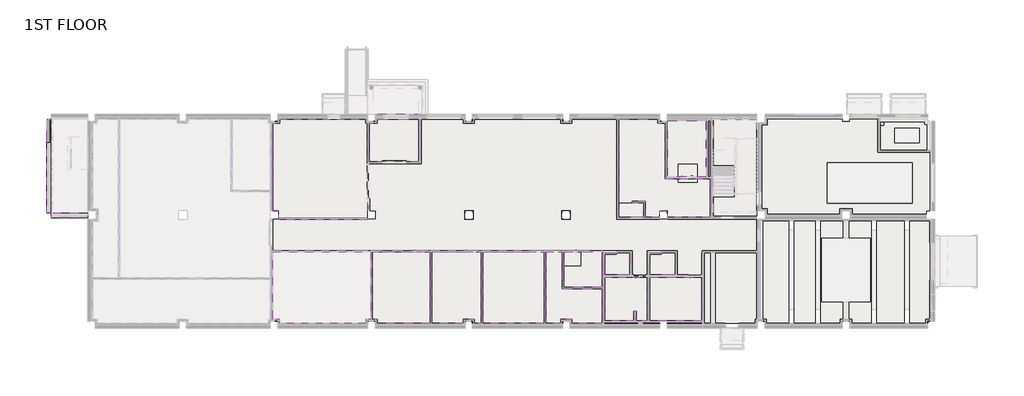
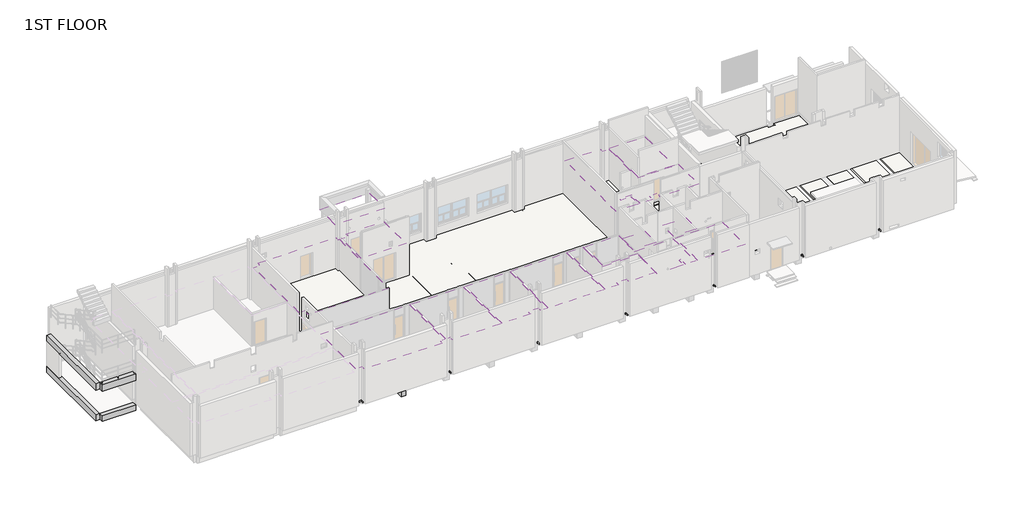
# One storey, part 8 of 15: 26 slabs, 15 coverings, 5 beams.
"""IFC4 building model written with IfcOpenShell, lengths in millimetres."""

from ifc_helpers import new_model, si_unit, frame, origin, place, context, project, spatial, polyline, outline, extrude, faceted_brep, element, save

model = new_model("IFC4")

# Units and contexts
model_context = context("Model", 3, world=origin())
ifc_project = project(units=[si_unit("LENGTHUNIT", "METRE", prefix="MILLI")], contexts=[model_context])

# Site, building, storey
site = spatial("IfcSite", under=ifc_project)
building = spatial("IfcBuilding", under=site)
storey = spatial("IfcBuildingStorey", under=building, Name="1ST FLOOR", Elevation=4800.0)

# Beams
placement = place(None, origin())
element("IfcBeam", 1, ObjectType="RC Beam_Rectangular : H_SB_AR S16_TG-UG_450x800_1B1A", at=placement, inside=storey, context=model_context, shape_type="Brep", body=[
    faceted_brep([(18775.0, -16900.0, 4800.0), (19225.0, -16900.0, 4800.0), (19225.0, -8350.0, 4800.0), (18775.0, -8350.0, 4800.0), (19225.0, -16900.0, 4650.0), (19225.0, -16900.0, 4000.0), (19225.0, -8350.0, 4000.0), (19225.0, -8350.0, 4650.0), (18775.0, -16900.0, 4000.0), (18775.0, -8350.0, 4000.0), (18775.0, -8350.0, 4650.0), (18775.0, -16900.0, 4650.0)], [[[0, 1, 2, 3]], [[2, 1, 4, 5, 6, 7]], [[5, 8, 9, 6]], [[0, 3, 10, 9, 8, 11]], [[1, 0, 11, 8, 5, 4]], [[3, 2, 7, 6, 9, 10]]]),
])
element("IfcBeam", 2, ObjectType="RC Beam_Rectangular : H_SB_AR S16_RC Beam-AG_400x530_SG1A", at=placement, inside=storey, context=model_context, shape_type="Brep", body=[
    faceted_brep([(-300.0, -8200.0, 4630.0), (-300.0, -7800.0, 4630.0), (-3300.0, -7800.0, 4630.0), (-3300.0, -8200.0, 4630.0), (-300.0, -8200.0, 4100.0), (-3300.0, -8200.0, 4100.0), (-300.0, -7800.0, 4100.0), (-3300.0, -7800.0, 4100.0), (-300.0, -7800.0, 4430.0), (-3300.0, -7800.0, 4430.0)], [[[0, 1, 2, 3]], [[4, 0, 3, 5]], [[6, 4, 5, 7]], [[1, 8, 6, 7, 9, 2]], [[1, 0, 4, 6, 8]], [[2, 9, 7, 5, 3]]]),
])
element("IfcBeam", 3, ObjectType="RC Beam_Rectangular : H_SB_AR S16_RC Beam-AG_400x600_SG2", at=placement, inside=storey, context=model_context, shape_type="Brep", body=[
    faceted_brep([(-3700.0, -7800.0, 4630.0), (-3300.0, -7800.0, 4630.0), (-3300.0, -100.0, 4630.0), (-3450.0, -100.0, 4630.0), (-3700.0, -100.0, 4630.0), (-3700.0, -2000.0, 4630.0), (-3700.0, -7800.0, 4030.0), (-3700.0, -100.0, 4030.0), (-3300.0, -7800.0, 4030.0), (-3300.0, -100.0, 4030.0), (-3300.0, -7800.0, 4430.0), (-3300.0, -100.0, 4430.0)], [[[0, 1, 2, 3, 4, 5]], [[6, 0, 5, 4, 7]], [[8, 6, 7, 9]], [[1, 10, 8, 9, 11, 2]], [[1, 0, 6, 8, 10]], [[2, 11, 9, 7, 4, 3]]]),
])
element("IfcBeam", 4, ObjectType="RC Beam_Rectangular : H_SB_AR S16_RC Beam-AG_400x600_SWG2", at=placement, inside=storey, context=model_context, shape_type="Brep", body=[
    faceted_brep([(-3300.0, -100.0, 7590.0), (-3450.0, -100.0, 7590.0), (-3700.0, -100.0, 7590.0), (-3700.0, -2000.0, 7590.0), (-3700.0, -7800.0, 7590.0), (-3300.0, -7800.0, 7590.0), (-3300.0, -100.0, 6990.0), (-3300.0, -7800.0, 6990.0), (-3700.0, -100.0, 6990.0), (-3450.0, -100.0, 6990.0), (-3700.0, -7800.0, 6990.0), (-3700.0, -2000.0, 6990.0)], [[[0, 1, 2, 3, 4, 5]], [[6, 0, 5, 7]], [[8, 9, 6, 7, 10, 11]], [[2, 8, 11, 10, 4, 3]], [[4, 10, 7, 5]], [[2, 1, 0, 6, 9, 8]]]),
])
element("IfcBeam", 5, ObjectType="RC Beam_Rectangular : H_SB_AR S16_RC Beam-AG_400x600_SG1", at=placement, inside=storey, context=model_context, shape_type="SweptSolid", body=[
    extrude(outline(polyline([(-300.0, -7800.0), (-300.0, -8200.0), (-3300.0, -8200.0), (-3300.0, -7800.0), (-300.0, -7800.0)])), frame((0.0, 0.0, 6990.0), z_axis=(0.0, 0.0, 1.0), x_axis=(1.0, 0.0, 0.0)), (0.0, 0.0, 1.0), 600.0),
])

# Coverings
element("IfcCovering", 6, ObjectType="H_CE_AR_B09_2L Gypsum Board_T Bar_9T_C4", at=placement, inside=storey, context=model_context, shape_type="SweptSolid", body=[
    extrude(outline(polyline([(22536.0, -114.0), (22536.0, -464.0), (22649.9999955, -464.0), (22649.9999955, -8250.0), (15400.0000001, -8250.0), (15400.0000001, -7650.0), (14886.0, -7650.0), (14886.0, -464.0), (15464.0, -464.0), (15464.0, -114.0), (22536.0, -114.0)])), frame((0.0, 0.0, 7830.0), z_axis=(0.0, 0.0, 1.0), x_axis=(1.0, 0.0, 0.0)), (0.0, 0.0, 1.0), 19.0),
])
element("IfcCovering", 7, ObjectType="H_CE_AR_B09_Aluminum Spandrel_M Bar_0.8T_C9", at=placement, inside=storey, context=model_context, shape_type="SweptSolid", body=[
    extrude(outline(polyline([(22836.0, -464.0), (23464.0, -464.0), (23464.0, -114.0), (26907.0, -114.0), (26907.0, -3607.0), (22836.0, -3607.0), (22836.0, -464.0)])), frame((0.0, 0.0, 7830.0), z_axis=(0.0, 0.0, 1.0), x_axis=(1.0, 0.0, 0.0)), (0.0, 0.0, 1.0), 0.8),
])
element("IfcCovering", 8, ObjectType="H_CE_AR_B09_2L Gypsum Board_T Bar_9T_C4", at=placement, inside=storey, context=model_context, shape_type="SweptSolid", body=[
    extrude(outline(polyline([(43343.0, -114.0), (46536.0, -114.0), (46536.0, -464.0), (47132.0, -464.0), (47132.0, -4993.0), (50825.0, -4993.0), (50825.0, -8164.0), (47349.9999999, -8164.0), (47349.9999999, -7650.0), (46649.9999999, -7650.0), (46649.9999999, -8164.0), (45514.0, -8164.0), (45514.0, -6836.0), (44443.0, -6836.0), (44443.0, -6964.0), (45386.0, -6964.0), (45386.0, -8164.0), (43343.0, -8164.0), (43343.0, -114.0)])), frame((0.0, 0.0, 7910.0), z_axis=(0.0, 0.0, 1.0), x_axis=(1.0, 0.0, 0.0)), (0.0, 0.0, 1.0), 19.0),
])
element("IfcCovering", 9, ObjectType="H_CE_AR_B09_SMC Ceiling_T Bar_300x300x0.8T_C6", at=placement, inside=storey, context=model_context, shape_type="SweptSolid", body=[
    extrude(outline(polyline([(50525.0, -4825.0), (47300.0, -4825.0), (47300.0, -250.0), (50525.0, -250.0), (50525.0, -4825.0)])), frame((0.0, 0.0, 7800.0), z_axis=(0.0, 0.0, 1.0), x_axis=(1.0, 0.0, 0.0)), (0.0, 0.0, 1.0), 0.8),
])
element("IfcCovering", 10, ObjectType="H_CE_AR_B09_2L Gypsum Board_T Bar_9T_C4", at=placement, inside=storey, context=model_context, shape_type="SweptSolid", body=[
    extrude(outline(polyline([(14886.0, -11007.0000083), (22936.0, -11007.0000083), (22936.0, -16536.0), (22536.0, -16536.0), (22536.0, -16886.0), (15464.0, -16886.0), (15464.0, -16536.0), (14886.0, -16536.0), (14886.0, -11007.0000083)])), frame((0.0, 0.0, 7830.0), z_axis=(0.0, 0.0, 1.0), x_axis=(1.0, 0.0, 0.0)), (0.0, 0.0, 1.0), 19.0),
])
element("IfcCovering", 11, ObjectType="H_CE_AR_B09_2L Gypsum Board_T Bar_9T_C4", at=placement, inside=storey, context=model_context, shape_type="SweptSolid", body=[
    extrude(outline(polyline([(23464.0, -16886.0), (23464.0, -16536.0), (23064.0, -16536.0), (23064.0, -11007.0), (27836.0, -11007.0), (27836.0, -16886.0), (23464.0, -16886.0)])), frame((0.0, 0.0, 7830.0), z_axis=(0.0, 0.0, 1.0), x_axis=(1.0, 0.0, 0.0)), (0.0, 0.0, 1.0), 19.0),
])
element("IfcCovering", 12, ObjectType="H_CE_AR_B09_Souns Absorbing Soft Fiber Board_T Bar_600x600x9T_C5", at=placement, inside=storey, context=model_context, shape_type="SweptSolid", body=[
    extrude(outline(polyline([(27964.0, -11007.0), (32036.0, -11007.0), (32036.0, -16886.0), (31464.0, -16886.0), (31464.0, -16536.0), (30536.0, -16536.0), (30536.0, -16886.0), (27964.0, -16886.0), (27964.0, -11007.0)])), frame((0.0, 0.0, 7830.0), z_axis=(0.0, 0.0, 1.0), x_axis=(1.0, 0.0, 0.0)), (0.0, 0.0, 1.0), 9.0),
])
element("IfcCovering", 13, ObjectType="H_CE_AR_B09_2L Gypsum Board_T Bar_9T_C4", at=placement, inside=storey, context=model_context, shape_type="SweptSolid", body=[
    extrude(outline(polyline([(37186.0, -11007.0), (37186.0, -16886.0), (32164.0, -16886.0), (32164.0, -11007.0), (37186.0, -11007.0)])), frame((0.0, 0.0, 7830.0), z_axis=(0.0, 0.0, 1.0), x_axis=(1.0, 0.0, 0.0)), (0.0, 0.0, 1.0), 19.0),
])
element("IfcCovering", 14, ObjectType="H_CE_AR_B09_Souns Absorbing Soft Fiber Board_T Bar_600x600x9T_C5", at=placement, inside=storey, context=model_context, shape_type="SweptSolid", body=[
    extrude(outline(polyline([(38686.0000001, -14064.0), (41957.0, -14064.0), (41957.0, -16886.0), (39464.0, -16886.0), (39464.0, -16536.0), (38536.0, -16536.0), (38536.0, -16886.0), (37314.0, -16886.0), (37314.0, -11007.0000083), (38686.0000001, -11007.0000083), (38686.0000001, -14064.0)])), frame((0.0, 0.0, 7830.0), z_axis=(0.0, 0.0, 1.0), x_axis=(1.0, 0.0, 0.0)), (0.0, 0.0, 1.0), 9.0),
])
element("IfcCovering", 15, ObjectType="H_CE_AR_B09_Souns Absorbing Soft Fiber Board_T Bar_600x600x9T_C5", at=placement, inside=storey, context=model_context, shape_type="SweptSolid", body=[
    extrude(outline(polyline([(41957.0, -11007.0), (41957.0, -13936.0), (38814.0000001, -13936.0), (38814.0000001, -11007.0), (41957.0, -11007.0)])), frame((0.0, 0.0, 7830.0), z_axis=(0.0, 0.0, 1.0), x_axis=(1.0, 0.0, 0.0)), (0.0, 0.0, 1.0), 9.0),
])
element("IfcCovering", 16, ObjectType="H_CE_AR_B09_2L Gypsum Board_T Bar_9T_C4", at=placement, inside=storey, context=model_context, shape_type="SweptSolid", body=[
    extrude(outline(polyline([(44245.0, -12895.0), (42155.0, -12895.0), (42155.0, -11105.0), (44245.0, -11105.0), (44245.0, -12895.0)])), frame((0.0, 0.0, 7500.0), z_axis=(0.0, 0.0, 1.0), x_axis=(1.0, 0.0, 0.0)), (0.0, 0.0, 1.0), 19.0),
])
element("IfcCovering", 17, ObjectType="H_CE_AR_B09_2L Gypsum Board_T Bar_9T_C4", at=placement, inside=storey, context=model_context, shape_type="SweptSolid", body=[
    extrude(outline(polyline([(45645.0, -13105.0), (45645.0, -16670.0), (44755.0, -16670.0), (44755.0, -15905.0), (44545.0, -15905.0), (44545.0, -16670.0), (42155.0, -16670.0), (42155.0, -13105.0), (45645.0, -13105.0)])), frame((0.0, 0.0, 7500.0), z_axis=(0.0, 0.0, 1.0), x_axis=(1.0, 0.0, 0.0)), (0.0, 0.0, 1.0), 19.0),
])
element("IfcCovering", 18, ObjectType="H_CE_AR_B09_2L Gypsum Board_T Bar_9T_C4", at=placement, inside=storey, context=model_context, shape_type="SweptSolid", body=[
    extrude(outline(polyline([(50145.0, -13105.0), (50145.0, -16670.0), (45855.0, -16670.0), (45855.0, -13105.0), (50145.0, -13105.0)])), frame((0.0, 0.0, 7500.0), z_axis=(0.0, 0.0, 1.0), x_axis=(1.0, 0.0, 0.0)), (0.0, 0.0, 1.0), 19.0),
])
element("IfcCovering", 19, ObjectType="H_CE_AR_B09_2L Gypsum Board_T Bar_9T_C4", at=placement, inside=storey, context=model_context, shape_type="SweptSolid", body=[
    extrude(outline(polyline([(47945.0, -11105.0000016), (47945.0, -12895.0), (45855.0, -12895.0), (45855.0, -11105.0000016), (47945.0, -11105.0000016)])), frame((0.0, 0.0, 7500.0), z_axis=(0.0, 0.0, 1.0), x_axis=(1.0, 0.0, 0.0)), (0.0, 0.0, 1.0), 19.0),
])
element("IfcCovering", 20, ObjectType="H_CE_AR_B09_Stainless Hairline Finish_3T", at=placement, inside=storey, context=model_context, shape_type="SweptSolid", body=[
    extrude(outline(polyline([(27247.0, 2747.0), (27247.0, 300.0), (22753.0, 300.0), (22753.0, 2747.0), (27247.0, 2747.0)]), holes=[polyline([(23150.0, 2650.0), (22850.0, 2650.0), (22850.0, 2350.0), (23150.0, 2350.0), (23150.0, 2650.0)]), polyline([(26850.0, 2650.0), (26850.0, 2350.0), (27150.0, 2350.0), (27150.0, 2650.0), (26850.0, 2650.0)])]), frame((0.0, 0.0, 8700.0), z_axis=(0.0, 0.0, 1.0), x_axis=(1.0, 0.0, 0.0)), (0.0, 0.0, 1.0), 3.0),
])

# Slabs
element("IfcSlab", 21, ObjectType="H_FL_AR_S17_RC Slab_T150_1S1", at=placement, inside=storey, context=model_context, shape_type="Brep", body=[
    faceted_brep([(18775.0, -100.0, 4650.0), (18775.0, -7850.0, 4650.0), (15400.0000001, -7850.0, 4650.0), (15400.0000001, -7650.0, 4650.0), (15100.0, -7650.0, 4650.0), (15100.0, -300.0, 4650.0), (15300.0, -300.0, 4650.0), (15300.0, -100.0, 4650.0), (18775.0, -7850.0, 4800.0), (18775.0, -100.0, 4800.0), (15300.0, -100.0, 4800.0), (15300.0, -300.0, 4800.0), (15100.0, -300.0, 4800.0), (15100.0, -7650.0, 4800.0), (15400.0000001, -7650.0, 4800.0), (15400.0000001, -7850.0, 4800.0)], [[[0, 1, 2, 3, 4, 5, 6, 7]], [[8, 9, 10, 11, 12, 13, 14, 15]], [[1, 0, 9, 8]], [[2, 1, 8, 15]], [[3, 2, 15, 14]], [[4, 3, 14, 13]], [[5, 4, 13, 12]], [[0, 7, 10, 9]], [[6, 5, 12, 11]], [[7, 6, 11, 10]]]),
    faceted_brep([(18775.0, -16900.0, 4650.0), (15300.0, -16900.0, 4650.0), (15300.0, -16700.0, 4650.0), (15100.0, -16700.0, 4650.0), (15100.0, -8350.0, 4650.0), (18775.0, -8350.0, 4650.0), (15300.0, -16900.0, 4800.0), (18775.0, -16900.0, 4800.0), (18775.0, -8350.0, 4800.0), (15400.0000001, -8350.0, 4800.0), (15100.0, -8350.0, 4800.0), (15100.0, -16700.0, 4800.0), (15300.0, -16700.0, 4800.0)], [[[0, 1, 2, 3, 4, 5]], [[6, 7, 8, 9, 10, 11, 12]], [[1, 0, 7, 6]], [[2, 1, 6, 12]], [[3, 2, 12, 11]], [[4, 3, 11, 10]], [[5, 4, 10, 9, 8]], [[0, 5, 8, 7]]]),
    faceted_brep([(22650.0000003, -7850.0, 4650.0), (19225.0, -7850.0, 4650.0), (19225.0, -100.0, 4650.0), (22700.0, -100.0, 4650.0), (22700.0, -7650.0, 4650.0), (22650.0000003, -7650.0, 4650.0), (19225.0, -7850.0, 4800.0), (22650.0000003, -7850.0, 4800.0), (22650.0000003, -7650.0, 4800.0), (22700.0, -7650.0, 4800.0), (22700.0, -300.0, 4800.0), (22700.0, -100.0, 4800.0), (19225.0, -100.0, 4800.0)], [[[0, 1, 2, 3, 4, 5]], [[6, 7, 8, 9, 10, 11, 12]], [[1, 0, 7, 6]], [[2, 1, 6, 12]], [[3, 2, 12, 11]], [[4, 3, 11, 10, 9]], [[5, 4, 9, 8]], [[0, 5, 8, 7]]]),
    faceted_brep([(19225.0, -8350.0, 4650.0), (22750.0, -8350.0, 4650.0), (22750.0, -16700.0, 4650.0), (22700.0, -16700.0, 4650.0), (22700.0, -16900.0, 4650.0), (19225.0, -16900.0, 4650.0), (22750.0, -8350.0, 4800.0), (22650.0, -8350.0, 4800.0), (19225.0, -8350.0, 4800.0), (19225.0, -16900.0, 4800.0), (22700.0, -16900.0, 4800.0), (22700.0, -16700.0, 4800.0), (22750.0, -16700.0, 4800.0)], [[[0, 1, 2, 3, 4, 5]], [[6, 7, 8, 9, 10, 11, 12]], [[1, 0, 8, 7, 6]], [[2, 1, 6, 12]], [[3, 2, 12, 11]], [[4, 3, 11, 10]], [[5, 4, 10, 9]], [[0, 5, 9, 8]]]),
    faceted_brep([(26775.0, -8350.0, 4650.0), (26775.0, -16900.0, 4650.0), (23300.0, -16900.0, 4650.0), (23300.0, -16700.0, 4650.0), (23250.0, -16700.0, 4650.0), (23250.0, -8350.0, 4650.0), (26775.0, -16900.0, 4800.0), (26775.0, -8350.0, 4800.0), (23350.0, -8350.0, 4800.0), (23250.0, -8350.0, 4800.0), (23250.0, -16700.0, 4800.0), (23300.0, -16700.0, 4800.0), (23300.0, -16900.0, 4800.0)], [[[0, 1, 2, 3, 4, 5]], [[6, 7, 8, 9, 10, 11, 12]], [[1, 0, 7, 6]], [[2, 1, 6, 12]], [[3, 2, 12, 11]], [[4, 3, 11, 10]], [[5, 4, 10, 9]], [[0, 5, 9, 8, 7]]]),
    faceted_brep([(23350.0000003, -7850.0, 4650.0), (23350.0000003, -7650.0, 4650.0), (23200.0, -7650.0, 4650.0), (23200.0, -300.0, 4650.0), (23300.0, -300.0, 4650.0), (23300.0, -100.0, 4650.0), (26775.0, -100.0, 4650.0), (26775.0, -7850.0, 4650.0), (23350.0000003, -7650.0, 4800.0), (23350.0000003, -7850.0, 4800.0), (26775.0, -7850.0, 4800.0), (26775.0, -100.0, 4800.0), (23300.0, -100.0, 4800.0), (23300.0, -300.0, 4800.0), (23200.0, -300.0, 4800.0), (23200.0, -7650.0, 4800.0)], [[[0, 1, 2, 3, 4, 5, 6, 7]], [[8, 9, 10, 11, 12, 13, 14, 15]], [[1, 0, 9, 8]], [[2, 1, 8, 15]], [[3, 2, 15, 14]], [[4, 3, 14, 13]], [[5, 4, 13, 12]], [[6, 5, 12, 11]], [[7, 6, 11, 10]], [[0, 7, 10, 9]]]),
    faceted_brep([(30700.0, -100.0, 4650.0), (30700.0, -300.0, 4650.0), (30750.0, -300.0, 4650.0), (30750.0, -7650.0, 4650.0), (30650.0000002, -7650.0, 4650.0), (30650.0000002, -7850.0, 4650.0), (27225.0, -7850.0, 4650.0), (27225.0, -100.0, 4650.0), (30700.0, -300.0, 4800.0), (30700.0, -100.0, 4800.0), (27225.0, -100.0, 4800.0), (27225.0, -7850.0, 4800.0), (30650.0000002, -7850.0, 4800.0), (30650.0000002, -7650.0, 4800.0), (30750.0, -7650.0, 4800.0), (30750.0, -300.0, 4800.0)], [[[0, 1, 2, 3, 4, 5, 6, 7]], [[8, 9, 10, 11, 12, 13, 14, 15]], [[1, 0, 9, 8]], [[2, 1, 8, 15]], [[3, 2, 15, 14]], [[4, 3, 14, 13]], [[5, 4, 13, 12]], [[6, 5, 12, 11]], [[7, 6, 11, 10]], [[0, 7, 10, 9]]]),
    faceted_brep([(30700.0, -16900.0, 4650.0), (27225.0, -16900.0, 4650.0), (27225.0, -8350.0, 4650.0), (30750.0, -8350.0, 4650.0), (30750.0, -16700.0, 4650.0), (30700.0, -16700.0, 4650.0), (27225.0, -16900.0, 4800.0), (30700.0, -16900.0, 4800.0), (30700.0, -16700.0, 4800.0), (30750.0, -16700.0, 4800.0), (30750.0, -8350.0, 4800.0), (30650.0, -8350.0, 4800.0), (27225.0, -8350.0, 4800.0)], [[[0, 1, 2, 3, 4, 5]], [[6, 7, 8, 9, 10, 11, 12]], [[1, 0, 7, 6]], [[2, 1, 6, 12]], [[3, 2, 12, 11, 10]], [[4, 3, 10, 9]], [[5, 4, 9, 8]], [[0, 5, 8, 7]]]),
    faceted_brep([(31300.0, -16900.0, 4650.0), (31300.0, -16700.0, 4650.0), (31250.0, -16700.0, 4650.0), (31250.0, -8350.0, 4650.0), (34775.0, -8350.0, 4650.0), (34775.0, -16900.0, 4650.0), (31300.0, -16700.0, 4800.0), (31300.0, -16900.0, 4800.0), (34775.0, -16900.0, 4800.0), (34775.0, -8350.0, 4800.0), (31350.0, -8350.0, 4800.0), (31250.0, -8350.0, 4800.0), (31250.0, -16700.0, 4800.0)], [[[0, 1, 2, 3, 4, 5]], [[6, 7, 8, 9, 10, 11, 12]], [[1, 0, 7, 6]], [[2, 1, 6, 12]], [[3, 2, 12, 11]], [[4, 3, 11, 10, 9]], [[5, 4, 9, 8]], [[0, 5, 8, 7]]]),
    faceted_brep([(31300.0, -100.0, 4650.0), (34775.0, -100.0, 4650.0), (34775.0, -7850.0, 4650.0), (31349.9999998, -7850.0, 4650.0), (31349.9999998, -7650.0, 4650.0), (31250.0, -7650.0, 4650.0), (31250.0, -300.0, 4650.0), (31300.0, -300.0, 4650.0), (34775.0, -100.0, 4800.0), (31300.0, -100.0, 4800.0), (31300.0, -300.0, 4800.0), (31250.0, -300.0, 4800.0), (31250.0, -7650.0, 4800.0), (31349.9999998, -7650.0, 4800.0), (31349.9999998, -7850.0, 4800.0), (34775.0, -7850.0, 4800.0)], [[[0, 1, 2, 3, 4, 5, 6, 7]], [[8, 9, 10, 11, 12, 13, 14, 15]], [[1, 0, 9, 8]], [[2, 1, 8, 15]], [[3, 2, 15, 14]], [[4, 3, 14, 13]], [[5, 4, 13, 12]], [[6, 5, 12, 11]], [[7, 6, 11, 10]], [[0, 7, 10, 9]]]),
    faceted_brep([(38700.0, -16900.0, 4650.0), (35225.0, -16900.0, 4650.0), (35225.0, -8350.0, 4650.0), (38750.0, -8350.0, 4650.0), (38750.0, -16700.0, 4650.0), (38700.0, -16700.0, 4650.0), (35225.0, -16900.0, 4800.0), (38700.0, -16900.0, 4800.0), (38700.0, -16700.0, 4800.0), (38750.0, -16700.0, 4800.0), (38750.0, -8350.0, 4800.0), (38650.0, -8350.0, 4800.0), (35225.0, -8350.0, 4800.0)], [[[0, 1, 2, 3, 4, 5]], [[6, 7, 8, 9, 10, 11, 12]], [[1, 0, 7, 6]], [[2, 1, 6, 12]], [[3, 2, 12, 11, 10]], [[4, 3, 10, 9]], [[5, 4, 9, 8]], [[0, 5, 8, 7]]]),
    faceted_brep([(38700.0, -100.0, 4650.0), (38700.0, -300.0, 4650.0), (38750.0, -300.0, 4650.0), (38750.0, -7650.0, 4650.0), (38650.0000002, -7650.0, 4650.0), (38650.0000002, -7850.0, 4650.0), (35225.0, -7850.0, 4650.0), (35225.0, -100.0, 4650.0), (38700.0, -300.0, 4800.0), (38700.0, -100.0, 4800.0), (35225.0, -100.0, 4800.0), (35225.0, -7850.0, 4800.0), (38650.0000002, -7850.0, 4800.0), (38650.0000002, -7650.0, 4800.0), (38750.0, -7650.0, 4800.0), (38750.0, -300.0, 4800.0)], [[[0, 1, 2, 3, 4, 5, 6, 7]], [[8, 9, 10, 11, 12, 13, 14, 15]], [[1, 0, 9, 8]], [[2, 1, 8, 15]], [[3, 2, 15, 14]], [[4, 3, 14, 13]], [[5, 4, 13, 12]], [[6, 5, 12, 11]], [[7, 6, 11, 10]], [[0, 7, 10, 9]]]),
    faceted_brep([(39300.0, -16900.0, 4650.0), (39300.0, -16700.0, 4650.0), (39250.0, -16700.0, 4650.0), (39250.0, -8350.0, 4650.0), (41675.0, -8350.0, 4650.0), (41675.0, -16900.0, 4650.0), (39300.0, -16700.0, 4800.0), (39300.0, -16900.0, 4800.0), (41675.0, -16900.0, 4800.0), (41675.0, -8350.0, 4800.0), (39350.0, -8350.0, 4800.0), (39250.0, -8350.0, 4800.0), (39250.0, -16700.0, 4800.0)], [[[0, 1, 2, 3, 4, 5]], [[6, 7, 8, 9, 10, 11, 12]], [[1, 0, 7, 6]], [[2, 1, 6, 12]], [[3, 2, 12, 11]], [[4, 3, 11, 10, 9]], [[5, 4, 9, 8]], [[0, 5, 8, 7]]]),
    faceted_brep([(39300.0, -100.0, 4650.0), (41675.0, -100.0, 4650.0), (41675.0, -7850.0, 4650.0), (39349.9999998, -7850.0, 4650.0), (39349.9999998, -7650.0, 4650.0), (39250.0, -7650.0, 4650.0), (39250.0, -300.0, 4650.0), (39300.0, -300.0, 4650.0), (41675.0, -100.0, 4800.0), (39300.0, -100.0, 4800.0), (39300.0, -300.0, 4800.0), (39250.0, -300.0, 4800.0), (39250.0, -7650.0, 4800.0), (39349.9999998, -7650.0, 4800.0), (39349.9999998, -7850.0, 4800.0), (41675.0, -7850.0, 4800.0)], [[[0, 1, 2, 3, 4, 5, 6, 7]], [[8, 9, 10, 11, 12, 13, 14, 15]], [[1, 0, 9, 8]], [[2, 1, 8, 15]], [[3, 2, 15, 14]], [[4, 3, 14, 13]], [[5, 4, 13, 12]], [[6, 5, 12, 11]], [[7, 6, 11, 10]], [[0, 7, 10, 9]]]),
    faceted_brep([(42125.0, -100.0, 4650.0), (44875.0, -100.0, 4650.0), (44875.0, -7850.0, 4650.0), (42125.0, -7850.0, 4650.0), (44875.0, -100.0, 4800.0), (42125.0, -100.0, 4800.0), (42125.0, -7850.0, 4800.0), (44875.0, -7850.0, 4800.0)], [[[0, 1, 2, 3]], [[4, 5, 6, 7]], [[1, 0, 5, 4]], [[2, 1, 4, 7]], [[3, 2, 7, 6]], [[0, 3, 6, 5]]]),
    faceted_brep([(46649.9999999, -7850.0, 4650.0), (45325.0, -7850.0, 4650.0), (45325.0, -100.0, 4650.0), (46700.0, -100.0, 4650.0), (46700.0, -300.0, 4650.0), (46800.0, -300.0, 4650.0), (46800.0, -7650.0, 4650.0), (46649.9999999, -7650.0, 4650.0), (45325.0, -7850.0, 4800.0), (46649.9999999, -7850.0, 4800.0), (46649.9999999, -7650.0, 4800.0), (46800.0, -7650.0, 4800.0), (46800.0, -300.0, 4800.0), (46700.0, -300.0, 4800.0), (46700.0, -100.0, 4800.0), (45325.0, -100.0, 4800.0)], [[[0, 1, 2, 3, 4, 5, 6, 7]], [[8, 9, 10, 11, 12, 13, 14, 15]], [[1, 0, 9, 8]], [[2, 1, 8, 15]], [[3, 2, 15, 14]], [[4, 3, 14, 13]], [[5, 4, 13, 12]], [[6, 5, 12, 11]], [[7, 6, 11, 10]], [[0, 7, 10, 9]]]),
    faceted_brep([(50825.0, -4825.0, 4650.0), (50825.0, -7850.0, 4650.0), (47349.9999999, -7850.0, 4650.0), (47300.0, -7850.0, 4650.0), (47300.0, -7650.0, 4650.0), (47300.0, -4825.0, 4650.0), (50825.0, -7850.0, 4800.0), (50825.0, -4825.0, 4800.0), (47300.0, -4825.0, 4800.0), (47300.0, -7650.0, 4800.0), (47300.0, -7850.0, 4800.0), (47349.9999999, -7850.0, 4800.0), (50825.0, -4825.0, 4700.0), (47300.0, -4825.0, 4700.0)], [[[0, 1, 2, 3, 4, 5]], [[6, 7, 8, 9, 10, 11]], [[1, 0, 12, 7, 6]], [[3, 2, 1, 6, 11, 10]], [[5, 4, 3, 10, 9, 8, 13]], [[0, 5, 13, 8, 7, 12]]]),
    faceted_brep([(54700.0, -8350.0, 4650.0), (54700.0, -16900.0, 4650.0), (51275.0, -16900.0, 4650.0), (51275.0, -8350.0, 4650.0), (54700.0, -16900.0, 4800.0), (54700.0, -16700.0, 4800.0), (54700.0, -8350.0, 4800.0), (51275.0, -8350.0, 4800.0), (51275.0, -16900.0, 4800.0)], [[[0, 1, 2, 3]], [[4, 5, 6, 7, 8]], [[1, 0, 6, 5, 4]], [[2, 1, 4, 8]], [[3, 2, 8, 7]], [[0, 3, 7, 6]]]),
    faceted_brep([(57275.0, -8350.0, 4650.0), (57275.0, -16900.0, 4650.0), (55300.0, -16900.0, 4650.0), (55300.0, -16700.0, 4650.0), (55200.0, -16700.0, 4650.0), (55200.0, -8350.0, 4650.0), (57275.0, -16900.0, 4800.0), (57275.0, -8350.0, 4800.0), (55200.0, -8350.0, 4800.0), (55200.0, -16700.0, 4800.0), (55300.0, -16700.0, 4800.0), (55300.0, -16900.0, 4800.0)], [[[0, 1, 2, 3, 4, 5]], [[6, 7, 8, 9, 10, 11]], [[1, 0, 7, 6]], [[2, 1, 6, 11]], [[3, 2, 11, 10]], [[4, 3, 10, 9]], [[5, 4, 9, 8]], [[0, 5, 8, 7]]]),
    faceted_brep([(59475.0, -8350.0, 4650.0), (59475.0, -16900.0, 4650.0), (57725.0, -16900.0, 4650.0), (57725.0, -8350.0, 4650.0), (59475.0, -16900.0, 4800.0), (59475.0, -8350.0, 4800.0), (57725.0, -8350.0, 4800.0), (57725.0, -16900.0, 4800.0)], [[[0, 1, 2, 3]], [[4, 5, 6, 7]], [[1, 0, 5, 4]], [[2, 1, 4, 7]], [[3, 2, 7, 6]], [[0, 3, 6, 5]]]),
    faceted_brep([(61750.0, -8350.0, 4650.0), (61750.0, -16700.0, 4650.0), (61700.0, -16700.0, 4650.0), (61700.0, -16900.0, 4650.0), (59925.0, -16900.0, 4650.0), (59925.0, -8350.0, 4650.0), (61750.0, -16700.0, 4800.0), (61750.0, -8350.0, 4800.0), (59925.0, -8350.0, 4800.0), (59925.0, -16900.0, 4800.0), (61700.0, -16900.0, 4800.0), (61700.0, -16700.0, 4800.0)], [[[0, 1, 2, 3, 4, 5]], [[6, 7, 8, 9, 10, 11]], [[1, 0, 7, 6]], [[2, 1, 6, 11]], [[3, 2, 11, 10]], [[4, 3, 10, 9]], [[5, 4, 9, 8]], [[0, 5, 8, 7]]]),
    faceted_brep([(62250.0, -8350.0, 4650.0), (64075.0, -8350.0, 4650.0), (64075.0, -16900.0, 4650.0), (62300.0, -16900.0, 4650.0), (62300.0, -16700.0, 4650.0), (62250.0, -16700.0, 4650.0), (64075.0, -8350.0, 4800.0), (62250.0, -8350.0, 4800.0), (62250.0, -16700.0, 4800.0), (62300.0, -16700.0, 4800.0), (62300.0, -16900.0, 4800.0), (64075.0, -16900.0, 4800.0)], [[[0, 1, 2, 3, 4, 5]], [[6, 7, 8, 9, 10, 11]], [[1, 0, 7, 6]], [[2, 1, 6, 11]], [[3, 2, 11, 10]], [[4, 3, 10, 9]], [[5, 4, 9, 8]], [[0, 5, 8, 7]]]),
    faceted_brep([(66775.0, -8350.0, 4650.0), (66775.0, -16900.0, 4650.0), (64525.0, -16900.0, 4650.0), (64525.0, -8350.0, 4650.0), (66775.0, -16900.0, 4800.0), (66775.0, -8350.0, 4800.0), (64525.0, -8350.0, 4800.0), (64525.0, -16900.0, 4800.0)], [[[0, 1, 2, 3]], [[4, 5, 6, 7]], [[1, 0, 5, 4]], [[2, 1, 4, 7]], [[3, 2, 7, 6]], [[0, 3, 6, 5]]]),
    faceted_brep([(68700.0, -16900.0, 4650.0), (67225.0, -16900.0, 4650.0), (67225.0, -8350.0, 4650.0), (68900.0, -8350.0, 4650.0), (68900.0, -16700.0, 4650.0), (68700.0, -16700.0, 4650.0), (67225.0, -16900.0, 4800.0), (68700.0, -16900.0, 4800.0), (68700.0, -16700.0, 4800.0), (68900.0, -16700.0, 4800.0), (68900.0, -8350.0, 4800.0), (67225.0, -8350.0, 4800.0)], [[[0, 1, 2, 3, 4, 5]], [[6, 7, 8, 9, 10, 11]], [[1, 0, 7, 6]], [[2, 1, 6, 11]], [[3, 2, 11, 10]], [[4, 3, 10, 9]], [[5, 4, 9, 8]], [[0, 5, 8, 7]]]),
    faceted_brep([(47250.0, -11075.0, 4650.0), (47250.0, -10675.0, 4650.0), (47250.0, -8350.0, 4650.0), (50825.0, -8350.0, 4650.0), (50825.0, -16900.0, 4650.0), (50575.0, -16900.0, 4650.0), (50175.0, -16900.0, 4650.0), (50175.0, -13075.0, 4650.0), (47975.0, -13075.0, 4650.0), (47975.0, -11075.0, 4650.0), (47250.0, -8350.0, 4800.0), (47250.0, -11075.0, 4800.0), (47975.0, -11075.0, 4800.0), (47975.0, -13075.0, 4800.0), (50175.0, -13075.0, 4800.0), (50175.0, -16900.0, 4800.0), (50825.0, -16900.0, 4800.0), (50825.0, -8350.0, 4800.0), (47350.0, -8350.0, 4800.0), (47250.0, -11075.0, 4700.0), (50175.0, -16900.0, 4700.0), (50175.0, -13075.0, 4700.0), (47975.0, -13075.0, 4700.0), (47975.0, -11075.0, 4700.0)], [[[0, 1, 2, 3, 4, 5, 6, 7, 8, 9]], [[10, 11, 12, 13, 14, 15, 16, 17, 18]], [[2, 1, 0, 19, 11, 10]], [[3, 2, 10, 18, 17]], [[4, 3, 17, 16]], [[6, 5, 4, 16, 15, 20]], [[7, 6, 20, 15, 14, 21]], [[8, 7, 21, 14, 13, 22]], [[9, 8, 22, 13, 12, 23]], [[0, 9, 23, 12, 11, 19]]]),
    faceted_brep([(46750.0, -8350.0, 4650.0), (46750.0, -10675.0, 4650.0), (46750.0, -11075.0, 4650.0), (45825.0, -11075.0, 4650.0), (45825.0, -13075.0, 4650.0), (45325.0, -13075.0, 4650.0), (45325.0, -12675.0, 4650.0), (45325.0, -8350.0, 4650.0), (46750.0, -11075.0, 4800.0), (46750.0, -8350.0, 4800.0), (46650.0, -8350.0, 4800.0), (45325.0, -8350.0, 4800.0), (45325.0, -13075.0, 4800.0), (45825.0, -13075.0, 4800.0), (45825.0, -11075.0, 4800.0), (46750.0, -11075.0, 4700.0), (45825.0, -11075.0, 4700.0), (45825.0, -13075.0, 4700.0), (45325.0, -13075.0, 4700.0)], [[[0, 1, 2, 3, 4, 5, 6, 7]], [[8, 9, 10, 11, 12, 13, 14]], [[2, 1, 0, 9, 8, 15]], [[3, 2, 15, 8, 14, 16]], [[4, 3, 16, 14, 13, 17]], [[5, 4, 17, 13, 12, 18]], [[7, 6, 5, 18, 12, 11]], [[0, 7, 11, 10, 9]]]),
    faceted_brep([(44875.0, -8350.0, 4650.0), (44875.0, -12675.0, 4650.0), (44875.0, -13075.0, 4650.0), (44275.0, -13075.0, 4650.0), (44275.0, -11075.0, 4650.0), (42125.0, -11075.0, 4650.0), (42125.0, -10675.0, 4650.0), (42125.0, -8350.0, 4650.0), (44875.0, -13075.0, 4800.0), (44875.0, -8350.0, 4800.0), (42125.0, -8350.0, 4800.0), (42125.0, -11075.0, 4800.0), (44275.0, -11075.0, 4800.0), (44275.0, -13075.0, 4800.0), (44875.0, -13075.0, 4700.0), (44275.0, -13075.0, 4700.0), (44275.0, -11075.0, 4700.0), (42125.0, -11075.0, 4700.0)], [[[0, 1, 2, 3, 4, 5, 6, 7]], [[8, 9, 10, 11, 12, 13]], [[2, 1, 0, 9, 8, 14]], [[3, 2, 14, 8, 13, 15]], [[4, 3, 15, 13, 12, 16]], [[5, 4, 16, 12, 11, 17]], [[7, 6, 5, 17, 11, 10]], [[0, 7, 10, 9]]]),
])
element("IfcSlab", 22, ObjectType="H_FL_AR_S17_RC Slab_T150_1S1", at=placement, inside=storey, context=model_context, shape_type="Brep", body=[
    faceted_brep([(50825.0, -100.0, 4550.0), (50825.0, -4825.0, 4550.0), (47300.0, -4825.0, 4550.0), (47300.0, -100.0, 4550.0), (50825.0, -100.0, 4700.0), (47300.0, -100.0, 4700.0), (47300.0, -4825.0, 4700.0), (50825.0, -4825.0, 4700.0), (50825.0, -4825.0, 4650.0), (47300.0, -4825.0, 4650.0)], [[[0, 1, 2, 3]], [[4, 5, 6, 7]], [[1, 0, 4, 7, 8]], [[2, 1, 8, 7, 6, 9]], [[3, 2, 9, 6, 5]], [[0, 3, 5, 4]]]),
])
element("IfcSlab", 23, ObjectType="H_FL_AR_S17_RC Slab_T150_GS1", at=placement, inside=storey, context=model_context, shape_type="Brep", body=[
    faceted_brep([(62312.0, -112.0, 4650.0), (64707.0, -112.0, 4650.0), (64707.0, -1062.0, 4650.0), (64707.0, -2743.0, 4650.0), (68888.0, -2743.0, 4650.0), (68888.0, -3093.0, 4650.0), (68888.0, -7638.0, 4650.0), (68588.0, -7638.0, 4650.0), (68588.0, -7938.0, 4650.0), (62362.0, -7938.0, 4650.0), (62362.0, -7638.0, 4650.0), (61638.0, -7638.0, 4650.0), (61638.0, -7938.0, 4650.0), (55362.0, -7938.0, 4650.0), (55362.0, -7638.0, 4650.0), (55062.0, -7638.0, 4650.0), (55062.0, -412.0, 4650.0), (55362.0, -412.0, 4650.0), (55362.0, -112.0, 4650.0), (61688.0, -112.0, 4650.0), (61688.0, -312.0, 4650.0), (62312.0, -312.0, 4650.0), (67450.0, -3700.0, 4650.0), (60450.0, -3700.0, 4650.0), (60450.0, -7000.0, 4650.0), (67450.0, -7000.0, 4650.0), (64707.0, -112.0, 4800.0), (62312.0, -112.0, 4800.0), (62312.0, -312.0, 4800.0), (61688.0, -312.0, 4800.0), (61688.0, -112.0, 4800.0), (55362.0, -112.0, 4800.0), (55362.0, -412.0, 4800.0), (55062.0, -412.0, 4800.0), (55062.0, -7638.0, 4800.0), (55362.0, -7638.0, 4800.0), (55362.0, -7938.0, 4800.0), (61638.0, -7938.0, 4800.0), (61638.0, -7638.0, 4800.0), (62362.0, -7638.0, 4800.0), (62362.0, -7938.0, 4800.0), (68588.0, -7938.0, 4800.0), (68588.0, -7638.0, 4800.0), (68888.0, -7638.0, 4800.0), (68888.0, -2743.0, 4800.0), (64707.0, -2743.0, 4800.0), (60450.0, -3700.0, 4800.0), (67450.0, -3700.0, 4800.0), (67450.0, -7000.0, 4800.0), (60450.0, -7000.0, 4800.0)], [[[0, 1, 2, 3, 4, 5, 6, 7, 8, 9, 10, 11, 12, 13, 14, 15, 16, 17, 18, 19, 20, 21], [22, 23, 24, 25]], [[26, 27, 28, 29, 30, 31, 32, 33, 34, 35, 36, 37, 38, 39, 40, 41, 42, 43, 44, 45], [46, 47, 48, 49]], [[1, 0, 27, 26]], [[6, 5, 4, 44, 43]], [[7, 6, 43, 42]], [[8, 7, 42, 41]], [[9, 8, 41, 40]], [[10, 9, 40, 39]], [[11, 10, 39, 38]], [[12, 11, 38, 37]], [[13, 12, 37, 36]], [[14, 13, 36, 35]], [[15, 14, 35, 34]], [[16, 15, 34, 33]], [[17, 16, 33, 32]], [[18, 17, 32, 31]], [[19, 18, 31, 30]], [[20, 19, 30, 29]], [[21, 20, 29, 28]], [[0, 21, 28, 27]], [[23, 22, 47, 46]], [[24, 23, 46, 49]], [[25, 24, 49, 48]], [[22, 25, 48, 47]], [[3, 2, 1, 26, 45]], [[4, 3, 45, 44]]]),
])
element("IfcSlab", 24, ObjectType="H_FL_AR_S17_RC Slab_T150_1S1", at=placement, inside=storey, context=model_context, shape_type="Brep", body=[
    faceted_brep([(47975.0, -11075.0, 4550.0), (47975.0, -13075.0, 4550.0), (50175.0, -13075.0, 4550.0), (50175.0, -16900.0, 4550.0), (47300.0, -16900.0, 4550.0), (47300.0, -16700.0, 4550.0), (47250.0, -16700.0, 4550.0), (47250.0, -11075.0, 4550.0), (47975.0, -11075.0, 4700.0), (47250.0, -11075.0, 4700.0), (47250.0, -16700.0, 4700.0), (47300.0, -16700.0, 4700.0), (47300.0, -16900.0, 4700.0), (50175.0, -16900.0, 4700.0), (50175.0, -13075.0, 4700.0), (47975.0, -13075.0, 4700.0), (47975.0, -11075.0, 4650.0), (47975.0, -13075.0, 4650.0), (50175.0, -13075.0, 4650.0), (50175.0, -16900.0, 4650.0), (47250.0, -11075.0, 4650.0)], [[[0, 1, 2, 3, 4, 5, 6, 7]], [[8, 9, 10, 11, 12, 13, 14, 15]], [[1, 0, 16, 8, 15, 17]], [[2, 1, 17, 15, 14, 18]], [[3, 2, 18, 14, 13, 19]], [[4, 3, 19, 13, 12]], [[5, 4, 12, 11]], [[6, 5, 11, 10]], [[7, 6, 10, 9, 20]], [[0, 7, 20, 9, 8, 16]]]),
    faceted_brep([(45325.0, -13075.0, 4550.0), (45825.0, -13075.0, 4550.0), (45825.0, -11075.0, 4550.0), (46750.0, -11075.0, 4550.0), (46750.0, -16700.0, 4550.0), (46700.0, -16700.0, 4550.0), (46700.0, -16900.0, 4550.0), (45325.0, -16900.0, 4550.0), (45325.0, -13075.0, 4700.0), (45325.0, -16900.0, 4700.0), (46700.0, -16900.0, 4700.0), (46700.0, -16700.0, 4700.0), (46750.0, -16700.0, 4700.0), (46750.0, -11075.0, 4700.0), (45825.0, -11075.0, 4700.0), (45825.0, -13075.0, 4700.0), (45325.0, -13075.0, 4650.0), (45825.0, -13075.0, 4650.0), (45825.0, -11075.0, 4650.0), (46750.0, -11075.0, 4650.0)], [[[0, 1, 2, 3, 4, 5, 6, 7]], [[8, 9, 10, 11, 12, 13, 14, 15]], [[1, 0, 16, 8, 15, 17]], [[2, 1, 17, 15, 14, 18]], [[3, 2, 18, 14, 13, 19]], [[4, 3, 19, 13, 12]], [[5, 4, 12, 11]], [[6, 5, 11, 10]], [[7, 6, 10, 9]], [[0, 7, 9, 8, 16]]]),
    faceted_brep([(44275.0, -11075.0, 4550.0), (44275.0, -13075.0, 4550.0), (44875.0, -13075.0, 4550.0), (44875.0, -16900.0, 4550.0), (42125.0, -16900.0, 4550.0), (42125.0, -11075.0, 4550.0), (44275.0, -11075.0, 4700.0), (42125.0, -11075.0, 4700.0), (42125.0, -16900.0, 4700.0), (44875.0, -16900.0, 4700.0), (44875.0, -13075.0, 4700.0), (44275.0, -13075.0, 4700.0), (44275.0, -11075.0, 4650.0), (44275.0, -13075.0, 4650.0), (44875.0, -13075.0, 4650.0), (42125.0, -11075.0, 4650.0)], [[[0, 1, 2, 3, 4, 5]], [[6, 7, 8, 9, 10, 11]], [[1, 0, 12, 6, 11, 13]], [[2, 1, 13, 11, 10, 14]], [[3, 2, 14, 10, 9]], [[4, 3, 9, 8]], [[5, 4, 8, 7, 15]], [[0, 5, 15, 7, 6, 12]]]),
])
element("IfcSlab", 25, ObjectType="H_FL_AR_S17_RC Slab_T200_SS1", at=placement, inside=storey, context=model_context, shape_type="SweptSolid", body=[
    extrude(outline(polyline([(54650.0, -100.0), (54650.0, -7950.0), (51225.0, -7950.0), (51225.0, -100.0), (54650.0, -100.0)])), frame((0.0, 0.0, 4600.0), z_axis=(0.0, 0.0, 1.0), x_axis=(1.0, 0.0, 0.0)), (0.0, 0.0, 1.0), 200.0),
])
element("IfcSlab", 26, ObjectType="H_FL_AR_S17_RC Slab_T150_GS1", at=placement, inside=storey, context=model_context, shape_type="Brep", body=[
    faceted_brep([(68688.0, -112.0, 4650.0), (68688.0, -312.0, 4650.0), (68888.0, -312.0, 4650.0), (68888.0, -2393.0, 4650.0), (68888.0, -2743.0, 4650.0), (64707.0, -2743.0, 4650.0), (64707.0, -1062.0, 4650.0), (64707.0, -112.0, 4650.0), (65257.0, -112.0, 4650.0), (65557.0, -112.0, 4650.0), (64807.0, -612.0, 4650.0), (65107.0, -612.0, 4650.0), (65107.0, -312.0, 4650.0), (64807.0, -312.0, 4650.0), (68688.0, -112.0, 4800.0), (68488.0, -112.0, 4800.0), (64707.0, -112.0, 4800.0), (64707.0, -2743.0, 4800.0), (68888.0, -2743.0, 4800.0), (68888.0, -312.0, 4800.0), (68688.0, -312.0, 4800.0), (64807.0, -612.0, 4800.0), (64807.0, -312.0, 4800.0), (65107.0, -312.0, 4800.0), (65107.0, -612.0, 4800.0)], [[[0, 1, 2, 3, 4, 5, 6, 7, 8, 9], [10, 11, 12, 13]], [[14, 15, 16, 17, 18, 19, 20], [21, 22, 23, 24]], [[1, 0, 14, 20]], [[2, 1, 20, 19]], [[4, 3, 2, 19, 18]], [[5, 4, 18, 17]], [[7, 6, 5, 17, 16]], [[0, 9, 8, 7, 16, 15, 14]], [[11, 10, 21, 24]], [[12, 11, 24, 23]], [[13, 12, 23, 22]], [[10, 13, 22, 21]]]),
])
element("IfcSlab", 27, ObjectType="H_FL_AR_B07_Wood Tile_600x600xT3_F8", at=placement, inside=storey, context=model_context, shape_type="SweptSolid", body=[
    extrude(outline(polyline([(15464.0, -464.0), (15464.0, -114.0), (22536.0, -114.0), (22536.0, -464.0), (22650.0, -464.0), (22650.0, -3793.0), (22749.9999955, -3793.0), (22749.9999955, -7650.0), (22650.0, -7650.0), (22650.0, -8350.0), (15400.0000001, -8350.0), (15400.0000001, -7650.0), (14886.0, -7650.0), (14886.0, -464.0), (15464.0, -464.0)])), frame((0.0, 0.0, 4800.0), z_axis=(0.0, 0.0, 1.0), x_axis=(1.0, 0.0, 0.0)), (0.0, 0.0, 1.0), 30.0),
])
element("IfcSlab", 28, ObjectType="H_FL_AR_B07_Deco Tile_600x600xT3", at=placement, inside=storey, context=model_context, shape_type="SweptSolid", body=[
    extrude(outline(polyline([(23350.0000003, -8350.0), (23350.0000003, -7650.0), (22749.9999955, -7650.0), (22749.9999955, -3793.0), (27093.0, -3793.0), (27093.0, -114.0), (30536.0, -114.0), (30536.0, -464.0), (31464.0, -464.0), (31464.0, -114.0), (38536.0, -114.0), (38536.0, -464.0), (39464.0, -464.0), (39464.0, -114.0), (43157.0, -114.0), (43157.0, -8350.0), (54650.0, -8350.0), (54650.0, -10907.0), (50157.0, -10907.0), (50157.0, -12907.0), (48143.0, -12907.0), (48143.0, -10907.0), (45657.0, -10907.0), (45657.0, -12907.0), (44443.0, -12907.0), (44443.0, -10907.0000083), (14886.0, -10907.0000083), (14886.0, -8350.0), (23350.0000003, -8350.0)]), holes=[polyline([(31350.0000002, -7650.0), (30649.9999999, -7650.0), (30649.9999999, -8350.0), (31350.0000002, -8350.0), (31350.0000002, -7650.0)]), polyline([(39349.9999999, -7650.0), (38649.9999999, -7650.0), (38649.9999999, -8350.0), (39349.9999999, -8350.0), (39349.9999999, -7650.0)])]), frame((0.0, 0.0, 4800.0), z_axis=(0.0, 0.0, 1.0), x_axis=(1.0, 0.0, 0.0)), (0.0, 0.0, 1.0), 30.0),
])
element("IfcSlab", 29, ObjectType="H_FL_AR_B07_Polishing Tile_600x600xT3", at=placement, inside=storey, context=model_context, shape_type="SweptSolid", body=[
    extrude(outline(polyline([(22836.0, -464.0), (23464.0, -464.0), (23464.0, -114.0), (26907.0, -114.0), (26907.0, -3607.0), (22836.0, -3607.0), (22836.0, -464.0)])), frame((0.0, 0.0, 4800.0), z_axis=(0.0, 0.0, 1.0), x_axis=(1.0, 0.0, 0.0)), (0.0, 0.0, 1.0), 30.0),
])
element("IfcSlab", 30, ObjectType="H_FL_AR_B07_Wood Tile_600x600xT3_F8", at=placement, inside=storey, context=model_context, shape_type="SweptSolid", body=[
    extrude(outline(polyline([(23064.0, -11007.0), (23000.0, -11007.0), (23000.0, -10907.0000083), (27900.0, -10907.0000083), (27900.0, -11007.0), (27836.0, -11007.0), (27836.0, -16886.0), (23464.0, -16886.0), (23464.0, -16536.0), (23064.0, -16536.0), (23064.0, -11007.0)])), frame((0.0, 0.0, 4800.0), z_axis=(0.0, 0.0, 1.0), x_axis=(1.0, 0.0, 0.0)), (0.0, 0.0, 1.0), 30.0),
])
element("IfcSlab", 31, ObjectType="H_FL_AR_B07_Deco Tile_600x600xT3", at=placement, inside=storey, context=model_context, shape_type="SweptSolid", body=[
    extrude(outline(polyline([(32100.0, -10907.0000083), (32100.0, -11007.0), (32036.0, -11007.0), (32036.0, -16886.0), (31464.0, -16886.0), (31464.0, -16536.0), (30536.0, -16536.0), (30536.0, -16886.0), (27964.0, -16886.0), (27964.0, -11007.0), (27900.0, -11007.0), (27900.0, -10907.0000083), (32100.0, -10907.0000083)])), frame((0.0, 0.0, 4800.0), z_axis=(0.0, 0.0, 1.0), x_axis=(1.0, 0.0, 0.0)), (0.0, 0.0, 1.0), 30.0),
])
element("IfcSlab", 32, ObjectType="H_FL_AR_B07_Capet Tile_600x600xT3", at=placement, inside=storey, context=model_context, shape_type="SweptSolid", body=[
    extrude(outline(polyline([(37250.0, -10907.0000083), (37250.0, -11007.0), (37186.0, -11007.0), (37186.0, -16886.0), (32164.0, -16886.0), (32164.0, -11007.0), (32100.0, -11007.0), (32100.0, -10907.0000083), (37250.0, -10907.0000083)])), frame((0.0, 0.0, 4800.0), z_axis=(0.0, 0.0, 1.0), x_axis=(1.0, 0.0, 0.0)), (0.0, 0.0, 1.0), 30.0),
])
element("IfcSlab", 33, ObjectType="H_FL_AR_B07_Deco Tile_600x600xT3", at=placement, inside=storey, context=model_context, shape_type="SweptSolid", body=[
    extrude(outline(polyline([(37314.0, -11007.0), (37250.0, -11007.0), (37250.0, -10907.0000083), (38750.0000001, -10907.0000083), (38750.0000001, -11007.0), (38686.0000001, -11007.0), (38686.0000001, -14064.0), (41957.0, -14064.0), (41957.0, -16886.0), (39464.0, -16886.0), (39464.0, -16536.0), (38536.0, -16536.0), (38536.0, -16886.0), (37314.0, -16886.0), (37314.0, -11007.0)])), frame((0.0, 0.0, 4800.0), z_axis=(0.0, 0.0, 1.0), x_axis=(1.0, 0.0, 0.0)), (0.0, 0.0, 1.0), 30.0),
])
element("IfcSlab", 34, ObjectType="H_FL_AR_B07_Wood Tile_600x600xT110_F8", at=placement, inside=storey, context=model_context, shape_type="SweptSolid", body=[
    extrude(outline(polyline([(41957.0, -10907.0000083), (41957.0, -13936.0), (38814.0000001, -13936.0), (38814.0000001, -12200.0), (40250.0, -12200.0), (40250.0, -10907.0000083), (41957.0, -10907.0000083)])), frame((0.0, 0.0, 4800.0), z_axis=(0.0, 0.0, 1.0), x_axis=(1.0, 0.0, 0.0)), (0.0, 0.0, 1.0), 110.0),
])
element("IfcSlab", 35, ObjectType="H_FL_AR_B07_Non-Slip Ceramic Tile_L Waterproof_300x300xT4", at=placement, inside=storey, context=model_context, shape_type="SweptSolid", body=[
    extrude(outline(polyline([(44245.0, -11105.0), (44245.0, -12895.0), (42155.0, -12895.0), (42155.0, -11105.0), (44245.0, -11105.0)])), frame((0.0, 0.0, 4700.0), z_axis=(0.0, 0.0, 1.0), x_axis=(1.0, 0.0, 0.0)), (0.0, 0.0, 1.0), 100.0),
])
element("IfcSlab", 36, ObjectType="H_FL_AR_B07_Non-Slip Ceramic Tile_L Waterproof_300x300xT4", at=placement, inside=storey, context=model_context, shape_type="SweptSolid", body=[
    extrude(outline(polyline([(45645.0, -13105.0), (45645.0, -16670.0), (44755.0, -16670.0), (44755.0, -15905.0), (44545.0, -15905.0), (44545.0, -16670.0), (42155.0, -16670.0), (42155.0, -13105.0), (45645.0, -13105.0)])), frame((0.0, 0.0, 4700.0), z_axis=(0.0, 0.0, 1.0), x_axis=(1.0, 0.0, 0.0)), (0.0, 0.0, 1.0), 100.0),
])
element("IfcSlab", 37, ObjectType="H_FL_AR_B07_Non-Slip Ceramic Tile_L Waterproof_300x300xT4", at=placement, inside=storey, context=model_context, shape_type="SweptSolid", body=[
    extrude(outline(polyline([(50145.0, -13105.0), (50145.0, -16670.0), (45855.0, -16670.0), (45855.0, -13105.0), (50145.0, -13105.0)])), frame((0.0, 0.0, 4700.0), z_axis=(0.0, 0.0, 1.0), x_axis=(1.0, 0.0, 0.0)), (0.0, 0.0, 1.0), 100.0),
])
element("IfcSlab", 38, ObjectType="H_FL_AR_B07_Non-Slip Ceramic Tile_L Waterproof_300x300xT4", at=placement, inside=storey, context=model_context, shape_type="SweptSolid", body=[
    extrude(outline(polyline([(47945.0, -11105.0000016), (47945.0, -12895.0), (45855.0, -12895.0), (45855.0, -11105.0000016), (47945.0, -11105.0000016)])), frame((0.0, 0.0, 4700.0), z_axis=(0.0, 0.0, 1.0), x_axis=(1.0, 0.0, 0.0)), (0.0, 0.0, 1.0), 100.0),
])
element("IfcSlab", 39, ObjectType="H_FL_AR_B07_Wood Tile_600x600xT110_F8", at=placement, inside=storey, context=model_context, shape_type="SweptSolid", body=[
    extrude(outline(polyline([(43343.0, -114.0), (46536.0, -114.0), (46536.0, -464.0), (47132.0, -464.0), (47132.0, -4993.0), (50825.0, -4993.0), (50825.0, -8164.0), (47349.9999999, -8164.0), (47349.9999999, -7650.0), (46649.9999999, -7650.0), (46649.9999999, -8164.0), (45386.0, -8164.0), (45386.0, -6964.0), (43343.0, -6964.0), (43343.0, -114.0)])), frame((0.0, 0.0, 4800.0), z_axis=(0.0, 0.0, 1.0), x_axis=(1.0, 0.0, 0.0)), (0.0, 0.0, 1.0), 110.0),
])
element("IfcSlab", 40, ObjectType="H_FL_AR_B07_Deco Tile_600x600xT3", at=placement, inside=storey, context=model_context, shape_type="SweptSolid", body=[
    extrude(outline(polyline([(45386.0, -6964.0), (45386.0, -8164.0), (43343.0, -8164.0), (43343.0, -6964.0), (45386.0, -6964.0)])), frame((0.0, 0.0, 4800.0), z_axis=(0.0, 0.0, 1.0), x_axis=(1.0, 0.0, 0.0)), (0.0, 0.0, 1.0), 30.0),
])
element("IfcSlab", 41, ObjectType="H_FL_AR_B07_Non-Slip Ceramic Tile_L Waterproof_300x300xT4", at=placement, inside=storey, context=model_context, shape_type="SweptSolid", body=[
    extrude(outline(polyline([(50495.0, -280.0), (50495.0, -4795.0), (47330.0, -4795.0), (47330.0, -280.0), (50495.0, -280.0)])), frame((0.0, 0.0, 4700.0), z_axis=(0.0, 0.0, 1.0), x_axis=(1.0, 0.0, 0.0)), (0.0, 0.0, 1.0), 100.0),
])
element("IfcSlab", 42, ObjectType="H_FL_AR_B07_Deco Tile_600x600xT3", at=placement, inside=storey, context=model_context, shape_type="SweptSolid", body=[
    extrude(outline(polyline([(54650.0, -114.0), (54650.0, -8100.0), (51075.0, -8100.0), (51075.0, -114.0), (54650.0, -114.0)])), frame((0.0, 0.0, 4800.0), z_axis=(0.0, 0.0, 1.0), x_axis=(1.0, 0.0, 0.0)), (0.0, 0.0, 1.0), 30.0),
])
element("IfcSlab", 43, ObjectType="H_FL_AR_B07_Wood Tile_600x600xT3_F8", at=placement, inside=storey, context=model_context, shape_type="SweptSolid", body=[
    extrude(outline(polyline([(40250.0, -10907.0000083), (40250.0, -12200.0), (38814.0000001, -12200.0), (38814.0000001, -11007.0), (38750.0000001, -11007.0), (38750.0000001, -10907.0000083), (40250.0, -10907.0000083)])), frame((0.0, 0.0, 4800.0), z_axis=(0.0, 0.0, 1.0), x_axis=(1.0, 0.0, 0.0)), (0.0, 0.0, 1.0), 30.0),
])
element("IfcSlab", 44, ObjectType="H_FL_AR_B07_Granite Tile_150x150xT30", at=placement, inside=storey, context=model_context, shape_type="SweptSolid", body=[
    extrude(outline(polyline([(49775.0, -4993.0), (49775.0, -5300.0), (48230.0, -5300.0), (48230.0, -4993.0), (49775.0, -4993.0)])), frame((0.0, 0.0, 4910.0), z_axis=(0.0, 0.0, 1.0), x_axis=(1.0, 0.0, 0.0)), (0.0, 0.0, 1.0), 90.0),
])
element("IfcSlab", 45, ObjectType="H_FL_AR_B07_Granite Tile_150x150xT30(Mortar_T170)", at=placement, inside=storey, context=model_context, shape_type="SweptSolid", body=[
    extrude(outline(polyline([(49775.0, -3800.0), (49775.0, -4795.0), (48230.0, -4795.0), (48230.0, -3800.0), (49775.0, -3800.0)])), frame((0.0, 0.0, 4800.0), z_axis=(0.0, 0.0, 1.0), x_axis=(1.0, 0.0, 0.0)), (0.0, 0.0, 1.0), 200.0),
])
element("IfcSlab", 46, ObjectType="H_FL_AR_S17_RC Slab_T300", at=placement, inside=storey, context=model_context, shape_type="Brep", body=[
    faceted_brep([(65257.0, -112.0, 4350.0), (65257.0, -762.0, 4350.0), (64657.0, -762.0, 4350.0), (64657.0, -112.0, 4350.0), (65257.0, -762.0, 4650.0), (65257.0, -112.0, 4650.0), (64707.0, -112.0, 4650.0), (64657.0, -112.0, 4650.0), (64657.0, -762.0, 4650.0), (64807.0, -312.0, 4650.0), (65107.0, -312.0, 4650.0), (65107.0, -612.0, 4650.0), (64807.0, -612.0, 4650.0), (65107.0, -312.0, 4500.0), (64807.0, -312.0, 4500.0), (64807.0, -612.0, 4500.0), (65107.0, -612.0, 4500.0)], [[[0, 1, 2, 3]], [[4, 5, 6, 7, 8], [9, 10, 11, 12]], [[1, 0, 5, 4]], [[2, 1, 4, 8]], [[3, 2, 8, 7]], [[0, 3, 7, 6, 5]], [[13, 14, 15, 16]], [[14, 13, 10, 9]], [[15, 14, 9, 12]], [[16, 15, 12, 11]], [[13, 16, 11, 10]]]),
])

save(model, "model.ifc")

# Revit data of these elements
# Type "RC Beam_Rectangular : H_SB_AR S16_TG-UG_450x800_1B1A"
#   Type Comments = "CV-UG"
#   중앙부 하부근 = ""
#   중앙부 상부근 = ""
#   중앙부 보조근 = ""
#   중앙부 늑근 = ""
#   외단부 하부근 = ""
#   외단부 상부근 = ""
#   외단부 보조근 = ""
#   외단부 늑근 = ""
#   부호 = "TG3"
#   내단부 하부근 = ""
#   내단부 상부근 = ""
#   내단부 보조근 = ""
#   내단부 늑근 = ""
#   ALL 하부근 = "3-D20"
#   ALL 상부근 = "3-D20"
#   ALL 보조근 = ""
#   ALL 늑근 = "2-D10 @120"
#   H_Rebar Ratio = 0.14
#   Width = 450 mm
#   Height = 800 mm
#   Length [instance default] = 1524 mm
#   b = 450 mm
#   h = 800 mm
#   hec_material3 [instance default] = none
#   hec_material2 [instance default] = none
#   hec_material1 [instance default] = none
#   Structural Material [instance default] = none
#   Assembly Code = ""
# Type "RC Beam_Rectangular : H_SB_AR S16_RC Beam-AG_400x530_SG1A"
#   Type Comments = "CV-AG"
#   중앙부 하부근 = ""
#   중앙부 상부근 = ""
#   중앙부 보조근 = ""
#   중앙부 늑근 = ""
#   외단부 하부근 = ""
#   외단부 상부근 = ""
#   외단부 보조근 = ""
#   외단부 늑근 = ""
#   부호 = "TG3"
#   내단부 하부근 = ""
#   내단부 상부근 = ""
#   내단부 보조근 = ""
#   내단부 늑근 = ""
#   ALL 하부근 = "3-D20"
#   ALL 상부근 = "3-D20"
#   ALL 보조근 = ""
#   ALL 늑근 = "2-D10 @120"
#   H_Rebar Ratio = 0.14
#   Width = 400 mm
#   Height = 530 mm
#   Length [instance default] = 1524 mm
#   b = 400 mm
#   h = 530 mm
#   hec_material3 [instance default] = none
#   hec_material2 [instance default] = none
#   hec_material1 [instance default] = none
#   Structural Material [instance default] = none
#   Assembly Code = ""
# Type "RC Beam_Rectangular : H_SB_AR S16_RC Beam-AG_400x600_SG2"
#   Type Comments = "CV-AG"
#   중앙부 하부근 = ""
#   중앙부 상부근 = ""
#   중앙부 보조근 = ""
#   중앙부 늑근 = ""
#   외단부 하부근 = ""
#   외단부 상부근 = ""
#   외단부 보조근 = ""
#   외단부 늑근 = ""
#   부호 = "TG3"
#   내단부 하부근 = ""
#   내단부 상부근 = ""
#   내단부 보조근 = ""
#   내단부 늑근 = ""
#   ALL 하부근 = "3-D20"
#   ALL 상부근 = "3-D20"
#   ALL 보조근 = ""
#   ALL 늑근 = "2-D10 @120"
#   H_Rebar Ratio = 0.14
#   Width = 400 mm
#   Height = 600 mm
#   Length [instance default] = 1524 mm
#   b = 400 mm
#   h = 600 mm
#   hec_material3 [instance default] = none
#   hec_material2 [instance default] = none
#   hec_material1 [instance default] = none
#   Structural Material [instance default] = none
#   Assembly Code = ""
# Type "RC Beam_Rectangular : H_SB_AR S16_RC Beam-AG_400x600_SWG2"
#   Type Comments = "CV-AG"
#   중앙부 하부근 = ""
#   중앙부 상부근 = ""
#   중앙부 보조근 = ""
#   중앙부 늑근 = ""
#   외단부 하부근 = ""
#   외단부 상부근 = ""
#   외단부 보조근 = ""
#   외단부 늑근 = ""
#   부호 = "TG3"
#   내단부 하부근 = ""
#   내단부 상부근 = ""
#   내단부 보조근 = ""
#   내단부 늑근 = ""
#   ALL 하부근 = "3-D20"
#   ALL 상부근 = "3-D20"
#   ALL 보조근 = ""
#   ALL 늑근 = "2-D10 @120"
#   H_Rebar Ratio = 0.14
#   Width = 400 mm
#   Height = 600 mm
#   Length [instance default] = 1524 mm
#   b = 400 mm
#   h = 600 mm
#   hec_material3 [instance default] = none
#   hec_material2 [instance default] = none
#   hec_material1 [instance default] = none
#   Structural Material [instance default] = none
#   Assembly Code = ""
# Type "RC Beam_Rectangular : H_SB_AR S16_RC Beam-AG_400x600_SG1"
#   Type Comments = "CV-AG"
#   중앙부 하부근 = ""
#   중앙부 상부근 = ""
#   중앙부 보조근 = ""
#   중앙부 늑근 = ""
#   외단부 하부근 = ""
#   외단부 상부근 = ""
#   외단부 보조근 = ""
#   외단부 늑근 = ""
#   부호 = "TG3"
#   내단부 하부근 = ""
#   내단부 상부근 = ""
#   내단부 보조근 = ""
#   내단부 늑근 = ""
#   ALL 하부근 = "3-D20"
#   ALL 상부근 = "3-D20"
#   ALL 보조근 = ""
#   ALL 늑근 = "2-D10 @120"
#   H_Rebar Ratio = 0.14
#   Width = 400 mm
#   Height = 600 mm
#   Length [instance default] = 1524 mm
#   b = 400 mm
#   h = 600 mm
#   hec_material3 [instance default] = none
#   hec_material2 [instance default] = none
#   hec_material1 [instance default] = none
#   Structural Material [instance default] = none
#   Assembly Code = ""
# Type "H_CE_AR_B09_2L Gypsum Board_T Bar_9T_C4"
#   built-in parameter 1002203 = 1 (stored number, unit not read)
#   built-in parameter 1002202 = 1 (stored number, unit not read)
